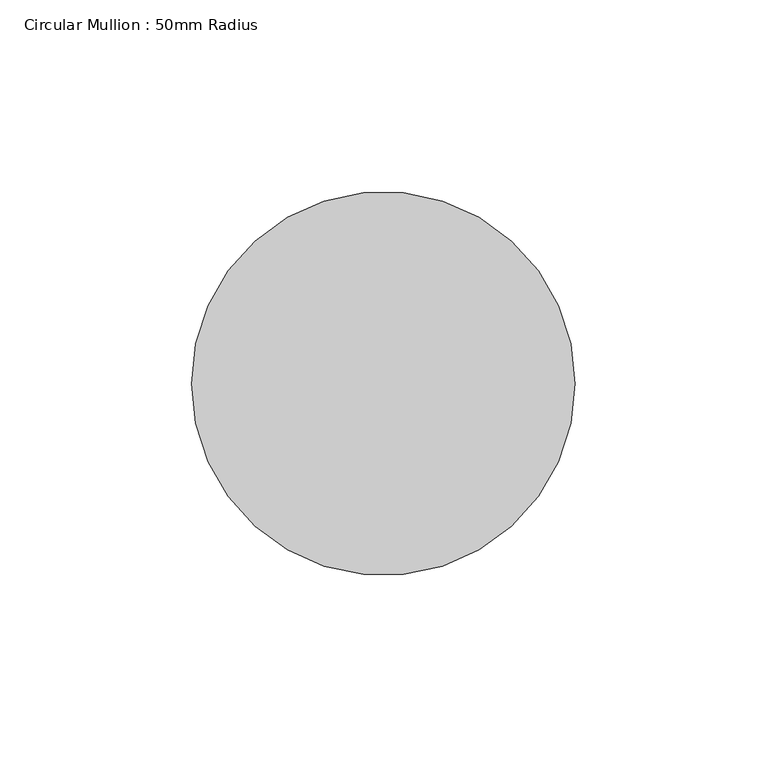
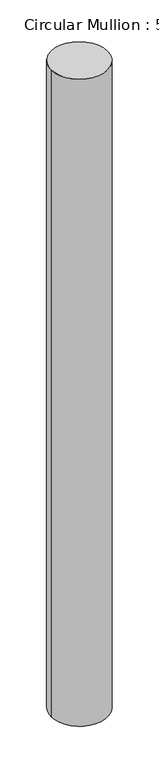
"""IFC4 building model written with IfcOpenShell, lengths in millimetres: member geometry, Circular Mullion : 50mm Radius."""

from ifc_helpers import new_model, si_unit, point, frame, origin, origin_2d, place, context, project, spatial, circle_curve, trimmed, segment, composite_curve, outline, extrude, source, transform, mapped, element, save


def circular_mullion_50mm_radius_62224457(model_context):
    return source(origin(), model_context, "Body", "SweptSolid", [
        extrude(outline(composite_curve([segment(trimmed(circle_curve(origin_2d(), 50.0), [point((50.0, 0.0))], [point((-50.0, 0.0))], False, "CARTESIAN"), True, "CONTINUOUS"), segment(trimmed(circle_curve(origin_2d(), 50.0), [point((-50.0, 0.0))], [point((50.0, 0.0))], False, "CARTESIAN"), True, "CONTINUOUS")], self_intersect=False)), frame((0.0, 0.0, -1206.3448853), z_axis=(0.0, 0.0, 1.0), x_axis=(1.0, 0.0, 0.0)), (0.0, 0.0, 1.0), 1206.3448853),
    ])


if __name__ == "__main__":
    model = new_model("IFC4")
    model_context = context("Model", 3, world=origin())
    ifc_project = project(units=[si_unit("LENGTHUNIT", "METRE", prefix="MILLI")], contexts=[model_context])
    site = spatial("IfcSite", under=ifc_project)
    building = spatial("IfcBuilding", under=site)
    placement = place(None, origin())
    circular_mullion_50mm_radius_shape = circular_mullion_50mm_radius_62224457(model_context)
    element("IfcMember", 1, ObjectType="Circular Mullion : 50mm Radius", at=placement, inside=building, context=model_context, shape_type="MappedRepresentation", body=[
        mapped(circular_mullion_50mm_radius_shape, transform((0.0, 0.0, 0.0), x_axis=(1.0, 0.0, 0.0), y_axis=(0.0, 1.0, 0.0), z_axis=(0.0, 0.0, 1.0))),
    ])
    save(model, "model.ifc")

# Revit data of these elements
# Type "Circular Mullion : 50mm Radius"
#   built-in parameter 1007350 = 0.164042 (stored number, unit not read)
# Element 1 (IfcMember, "Circular Mullion : 50mm Radius")
#   Materials on its faces: "Aluminium"
# Materials
#   "Aluminium": class "Metal", colour RGB 247 247 247, transparency 0, Description = "Aluminium 6061", Cost = 0
